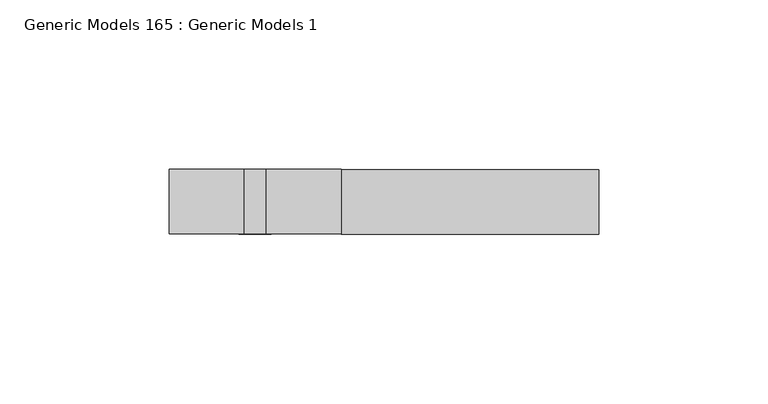
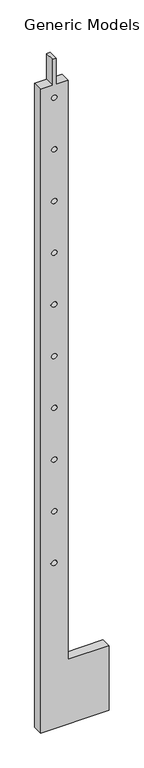
"""IFC4 building model written with IfcOpenShell, lengths in millimetres: proxy geometry, Generic Models 165 : Generic Models 1."""

from ifc_helpers import new_model, si_unit, point, frame, frame_2d, origin, place, context, project, spatial, polyline, circle_curve, trimmed, segment, composite_curve, outline, extrude, source, transform, mapped, element, save


def generic_models_165_generic_models_1_af1275b7(model_context):
    return source(origin(), model_context, "Body", "SweptSolid", [
        extrude(outline(polyline([(122933.4234874, -10313.8972239), (124071.6609874, -10313.8972239), (124071.6609874, -10336.1222239), (124122.4609874, -10336.1222239), (124122.4609874, -10342.4722239), (124071.6609874, -10342.4722239), (124071.6609874, -10364.6972239), (122806.4234874, -10364.6972239), (122806.4234874, -10237.6972239), (122933.4234874, -10237.6972239), (122933.4234874, -10313.8972239)]), holes=[composite_curve([segment(trimmed(circle_curve(frame_2d((123131.8609874, -10339.2972239)), 4.7625), [point((123131.8609874, -10344.0597239))], [point((123131.8609874, -10334.5347239))], True, "CARTESIAN"), True, "CONTINUOUS"), segment(trimmed(circle_curve(frame_2d((123131.8609874, -10339.2972239)), 4.7625), [point((123131.8609874, -10334.5347239))], [point((123131.8609874, -10344.0597239))], True, "CARTESIAN"), True, "CONTINUOUS")], self_intersect=False), composite_curve([segment(trimmed(circle_curve(frame_2d((123233.4609874, -10339.2972239)), 4.7625), [point((123233.4609874, -10344.0597239))], [point((123233.4609874, -10334.5347239))], True, "CARTESIAN"), True, "CONTINUOUS"), segment(trimmed(circle_curve(frame_2d((123233.4609874, -10339.2972239)), 4.7625), [point((123233.4609874, -10334.5347239))], [point((123233.4609874, -10344.0597239))], True, "CARTESIAN"), True, "CONTINUOUS")], self_intersect=False), composite_curve([segment(trimmed(circle_curve(frame_2d((123335.0609874, -10339.2972239)), 4.7625), [point((123335.0609874, -10344.0597239))], [point((123335.0609874, -10334.5347239))], True, "CARTESIAN"), True, "CONTINUOUS"), segment(trimmed(circle_curve(frame_2d((123335.0609874, -10339.2972239)), 4.7625), [point((123335.0609874, -10334.5347239))], [point((123335.0609874, -10344.0597239))], True, "CARTESIAN"), True, "CONTINUOUS")], self_intersect=False), composite_curve([segment(trimmed(circle_curve(frame_2d((123436.6609874, -10339.2972239)), 4.7625), [point((123436.6609874, -10344.0597239))], [point((123436.6609874, -10334.5347239))], True, "CARTESIAN"), True, "CONTINUOUS"), segment(trimmed(circle_curve(frame_2d((123436.6609874, -10339.2972239)), 4.7625), [point((123436.6609874, -10334.5347239))], [point((123436.6609874, -10344.0597239))], True, "CARTESIAN"), True, "CONTINUOUS")], self_intersect=False), composite_curve([segment(trimmed(circle_curve(frame_2d((123538.2609874, -10339.2972239)), 4.7625), [point((123538.2609874, -10344.0597239))], [point((123538.2609874, -10334.5347239))], True, "CARTESIAN"), True, "CONTINUOUS"), segment(trimmed(circle_curve(frame_2d((123538.2609874, -10339.2972239)), 4.7625), [point((123538.2609874, -10334.5347239))], [point((123538.2609874, -10344.0597239))], True, "CARTESIAN"), True, "CONTINUOUS")], self_intersect=False), composite_curve([segment(trimmed(circle_curve(frame_2d((123639.8609874, -10339.2972239)), 4.7625), [point((123639.8609874, -10344.0597239))], [point((123639.8609874, -10334.5347239))], True, "CARTESIAN"), True, "CONTINUOUS"), segment(trimmed(circle_curve(frame_2d((123639.8609874, -10339.2972239)), 4.7625), [point((123639.8609874, -10334.5347239))], [point((123639.8609874, -10344.0597239))], True, "CARTESIAN"), True, "CONTINUOUS")], self_intersect=False), composite_curve([segment(trimmed(circle_curve(frame_2d((123741.4609874, -10339.2972239)), 4.7625), [point((123741.4609874, -10344.0597239))], [point((123741.4609874, -10334.5347239))], True, "CARTESIAN"), True, "CONTINUOUS"), segment(trimmed(circle_curve(frame_2d((123741.4609874, -10339.2972239)), 4.7625), [point((123741.4609874, -10334.5347239))], [point((123741.4609874, -10344.0597239))], True, "CARTESIAN"), True, "CONTINUOUS")], self_intersect=False), composite_curve([segment(trimmed(circle_curve(frame_2d((123843.0609874, -10339.2972239)), 4.7625), [point((123843.0609874, -10344.0597239))], [point((123843.0609874, -10334.5347239))], True, "CARTESIAN"), True, "CONTINUOUS"), segment(trimmed(circle_curve(frame_2d((123843.0609874, -10339.2972239)), 4.7625), [point((123843.0609874, -10334.5347239))], [point((123843.0609874, -10344.0597239))], True, "CARTESIAN"), True, "CONTINUOUS")], self_intersect=False), composite_curve([segment(trimmed(circle_curve(frame_2d((123944.6609874, -10339.2972239)), 4.7625), [point((123944.6609874, -10344.0597239))], [point((123944.6609874, -10334.5347239))], True, "CARTESIAN"), True, "CONTINUOUS"), segment(trimmed(circle_curve(frame_2d((123944.6609874, -10339.2972239)), 4.7625), [point((123944.6609874, -10334.5347239))], [point((123944.6609874, -10344.0597239))], True, "CARTESIAN"), True, "CONTINUOUS")], self_intersect=False), composite_curve([segment(trimmed(circle_curve(frame_2d((124046.2609874, -10339.2972239)), 4.7625), [point((124046.2609874, -10344.0597239))], [point((124046.2609874, -10334.5347239))], True, "CARTESIAN"), True, "CONTINUOUS"), segment(trimmed(circle_curve(frame_2d((124046.2609874, -10339.2972239)), 4.7625), [point((124046.2609874, -10334.5347239))], [point((124046.2609874, -10344.0597239))], True, "CARTESIAN"), True, "CONTINUOUS")], self_intersect=False)]), frame((0.0, 542.6395048, 0.0), z_axis=(0.0, 1.0, 0.0), x_axis=(0.0, 0.0, 1.0)), (0.0, 0.0, 1.0), 19.05),
    ])


if __name__ == "__main__":
    model = new_model("IFC4")
    model_context = context("Model", 3, world=origin())
    ifc_project = project(units=[si_unit("LENGTHUNIT", "METRE", prefix="MILLI")], contexts=[model_context])
    site = spatial("IfcSite", under=ifc_project)
    building = spatial("IfcBuilding", under=site)
    placement = place(None, origin())
    generic_models_165_generic_models_1_shape = generic_models_165_generic_models_1_af1275b7(model_context)
    element("IfcBuildingElementProxy", 1, Name="Generic Models 165 : Generic Models 1", ObjectType="Generic Models 165 : Generic Models 1", at=placement, inside=building, context=model_context, shape_type="MappedRepresentation", body=[
        mapped(generic_models_165_generic_models_1_shape, transform((0.0, 0.0, 0.0), x_axis=(1.0, 0.0, 0.0), y_axis=(0.0, 1.0, 0.0), z_axis=(0.0, 0.0, 1.0))),
    ])
    save(model, "model.ifc")

# Revit data of these elements
# Element 1 (IfcBuildingElementProxy, "Generic Models 165 : Generic Models 1")
#   Materials on its faces: "_3/4\" x 1 1/2\" FLAT STOCK PAINTED STEEL POSTS"
# Materials
#   "_3/4\" x 1 1/2\" FLAT STOCK PAINTED STEEL POSTS": class "Generic", colour RGB 233 233 233, transparency 0, Cost = 0
